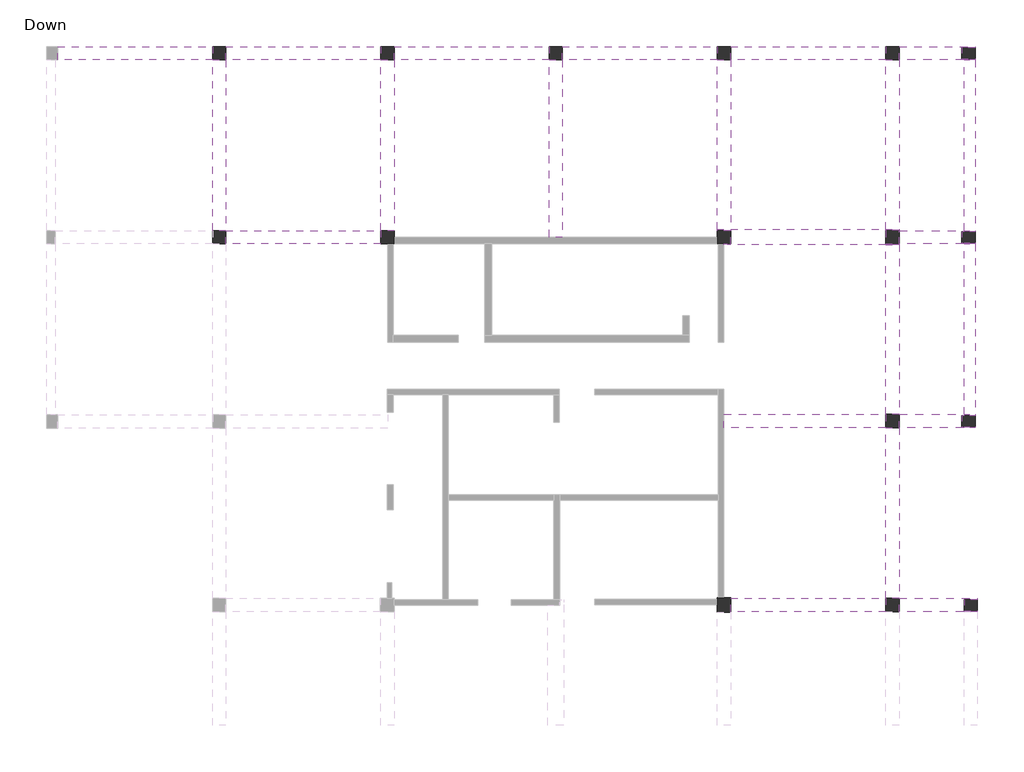
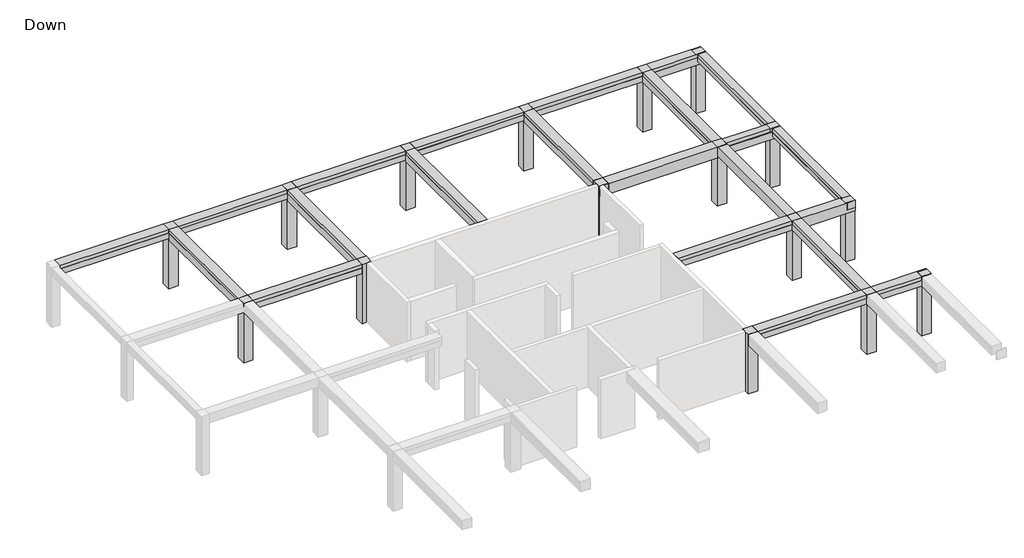
# One storey, part 2 of 2: 22 beams, 16 columns.
"""IFC4 building model written with IfcOpenShell, lengths in millimetres."""

from ifc_helpers import new_model, si_unit, frame, origin, origin_with_axes, place, context, project, spatial, polyline, outline, extrude, faceted_brep, element, save

model = new_model("IFC4")

# Units and contexts
model_context = context("Model", 3, world=origin())
ifc_project = project(units=[si_unit("LENGTHUNIT", "METRE", prefix="MILLI")], contexts=[model_context])

# Site, building, storey
site = spatial("IfcSite", under=ifc_project)
building = spatial("IfcBuilding", under=site)
storey = spatial("IfcBuildingStorey", under=building, Name="Down", Elevation=0.0)

# Beams
placement = place(None, origin())
element("IfcBeam", 1, ObjectType="Concrete Rectengular Beam : 50/50", at=placement, inside=storey, context=model_context, shape_type="Brep", body=[
    faceted_brep([(20278.3855721, 17336.6191558, 4000.0), (20278.3855721, 17386.6191558, 4000.0), (19788.3855721, 17386.6191558, 4000.0), (19788.3855721, 17336.6191558, 4000.0), (19778.3855721, 17386.6191558, 3500.0), (19778.3855721, 17336.6191558, 3500.0), (19778.3855721, 17336.6191558, 3770.0), (19778.3855721, 17386.6191558, 3770.0), (20278.3855721, 17336.6191558, 3500.0), (20278.3855721, 17386.6191558, 3500.0), (19788.3855721, 17336.6191558, 3770.0), (19788.3855721, 17386.6191558, 3770.0)], [[[0, 1, 2, 3]], [[4, 5, 6, 7]], [[8, 5, 4, 9]], [[0, 8, 9, 1]], [[5, 8, 0, 3, 10, 6]], [[9, 4, 7, 11, 2, 1]], [[10, 11, 7, 6]], [[11, 10, 3, 2]]]),
    faceted_brep([(20278.3855721, 25592.9632364, 3500.0), (19778.3855721, 25592.9632364, 3500.0), (19778.3855721, 25592.9632364, 3770.0), (19788.3855721, 25592.9632364, 3770.0), (19788.3855721, 25592.9632364, 4000.0), (20278.3855721, 25592.9632364, 4000.0), (19778.3855721, 17936.6191558, 3770.0), (19778.3855721, 17886.6191558, 3770.0), (19788.3855721, 17886.6191558, 3770.0), (19788.3855721, 17886.6191558, 4000.0), (20278.3855721, 17886.6191558, 4000.0), (19778.3855721, 17886.6191558, 3500.0), (20278.3855721, 17886.6191558, 3500.0), (19778.3855721, 17936.6191558, 3500.0), (20278.3855721, 17936.6191558, 3500.0)], [[[0, 1, 2, 3, 4, 5]], [[3, 2, 6, 7, 8]], [[4, 3, 8, 9]], [[10, 9, 8, 7, 11, 12]], [[10, 5, 4, 9]], [[1, 13, 11, 7, 6, 2]], [[1, 0, 14, 12, 11, 13]], [[0, 5, 10, 12, 14]]]),
])
element("IfcBeam", 2, ObjectType="Concrete Rectengular Beam : 50/50", at=placement, inside=storey, context=model_context, shape_type="Brep", body=[
    faceted_brep([(19778.3855721, 9081.6131842, 4000.0), (20278.3855721, 9081.6131842, 4000.0), (20278.3855721, 9131.6131842, 4000.0), (19778.3855721, 9131.6131842, 4000.0), (19778.3855721, 9081.6131842, 3500.0), (19778.3855721, 9131.6131842, 3500.0), (20278.3855721, 9081.6131842, 3500.0), (20278.3855721, 9131.6131842, 3500.0)], [[[0, 1, 2, 3]], [[4, 0, 3, 5]], [[6, 4, 5, 7]], [[1, 6, 7, 2]], [[1, 0, 4, 6]], [[3, 2, 7, 5]]]),
    faceted_brep([(20278.3855721, 9631.6131842, 4000.0), (19778.3855721, 9631.6131842, 4000.0), (19778.3855721, 9631.6131842, 3500.0), (20278.3855721, 9631.6131842, 3500.0), (20278.3855721, 17336.6191558, 4000.0), (19788.3855721, 17336.6191558, 4000.0), (19788.3855721, 9676.6131842, 4000.0), (19778.3855721, 9676.6131842, 4000.0), (19778.3855721, 9676.6131842, 3770.0), (19778.3855721, 9681.6131842, 3770.0), (19778.3855721, 17336.6191558, 3770.0), (19778.3855721, 17336.6191558, 3500.0), (19778.3855721, 9681.6131842, 3500.0), (20278.3855721, 17336.6191558, 3500.0), (20278.3855721, 9681.6131842, 3500.0), (19788.3855721, 17336.6191558, 3770.0), (19788.3855721, 9676.6131842, 3770.0)], [[[0, 1, 2, 3]], [[1, 0, 4, 5, 6, 7]], [[2, 1, 7, 8, 9, 10, 11, 12]], [[3, 2, 12, 11, 13, 14]], [[0, 3, 14, 13, 4]], [[13, 11, 10, 15, 5, 4]], [[8, 16, 15, 10, 9]], [[16, 6, 5, 15]], [[6, 16, 8, 7]]]),
])
element("IfcBeam", 3, ObjectType="Concrete Rectengular Beam : 60/60", at=placement, inside=storey, context=model_context, shape_type="SweptSolid", body=[
    extrude(outline(polyline([(26192.9632364, 3400.0), (25592.9632364, 3400.0), (25592.9632364, 3770.0), (25597.9632364, 3770.0), (25597.9632364, 4000.0), (26192.9632364, 4000.0), (26192.9632364, 3400.0)])), frame((-20894.7160223, 0.0, 0.0), z_axis=(1.0, 0.0, 0.0), x_axis=(0.0, 1.0, 0.0)), (0.0, 0.0, 1.0), 6950.9015474),
])
element("IfcBeam", 4, ObjectType="Concrete Rectengular Beam : 60/60", at=placement, inside=storey, context=model_context, shape_type="SweptSolid", body=[
    extrude(outline(polyline([(26192.9632364, 3400.0), (25592.9632364, 3400.0), (25592.9632364, 3770.0), (25597.9632364, 3770.0), (25597.9632364, 4000.0), (26192.9632364, 4000.0), (26192.9632364, 3400.0)])), frame((-13343.8144749, 0.0, 0.0), z_axis=(1.0, 0.0, 0.0), x_axis=(0.0, 1.0, 0.0)), (0.0, 0.0, 1.0), 6953.6558928),
])
element("IfcBeam", 5, ObjectType="Concrete Rectengular Beam : 60/60", at=placement, inside=storey, context=model_context, shape_type="SweptSolid", body=[
    extrude(outline(polyline([(26192.9632364, 3400.0), (25592.9632364, 3400.0), (25592.9632364, 3770.0), (25597.9632364, 3770.0), (25597.9632364, 4000.0), (26192.9632364, 4000.0), (26192.9632364, 3400.0)])), frame((-5790.1585821, 0.0, 0.0), z_axis=(1.0, 0.0, 0.0), x_axis=(0.0, 1.0, 0.0)), (0.0, 0.0, 1.0), 6947.2395979),
])
element("IfcBeam", 6, ObjectType="Concrete Rectengular Beam : 60/60", at=placement, inside=storey, context=model_context, shape_type="SweptSolid", body=[
    extrude(outline(polyline([(26192.9632364, 3400.0), (25592.9632364, 3400.0), (25592.9632364, 3770.0), (25597.9632364, 3770.0), (25597.9632364, 4000.0), (26192.9632364, 4000.0), (26192.9632364, 3400.0)])), frame((1757.0810158, 0.0, 0.0), z_axis=(1.0, 0.0, 0.0), x_axis=(0.0, 1.0, 0.0)), (0.0, 0.0, 1.0), 6946.2785308),
])
element("IfcBeam", 7, ObjectType="Concrete Rectengular Beam : 60/60", at=placement, inside=storey, context=model_context, shape_type="SweptSolid", body=[
    extrude(outline(polyline([(26192.9632364, 3400.0), (25592.9632364, 3400.0), (25592.9632364, 3770.0), (25597.9632364, 3770.0), (25597.9632364, 4000.0), (26192.9632364, 4000.0), (26192.9632364, 3400.0)])), frame((9303.3595467, 0.0, 0.0), z_axis=(1.0, 0.0, 0.0), x_axis=(0.0, 1.0, 0.0)), (0.0, 0.0, 1.0), 6958.5206647),
])
element("IfcBeam", 8, ObjectType="Concrete Rectengular Beam : 60/60", at=placement, inside=storey, context=model_context, shape_type="SweptSolid", body=[
    extrude(outline(polyline([(3400.0, 16261.8802114), (3400.0, 16861.8802114), (4000.0, 16861.8802114), (4000.0, 16266.8802114), (3770.0, 16266.8802114), (3770.0, 16261.8802114), (3400.0, 16261.8802114)])), frame((0.0, 1432.5009852, 0.0), z_axis=(0.0, 1.0, 0.0), x_axis=(0.0, 0.0, 1.0)), (0.0, 0.0, 1.0), 7649.112199),
])
element("IfcBeam", 9, ObjectType="Concrete Rectengular Beam : 60/60", at=placement, inside=storey, context=model_context, shape_type="SweptSolid", body=[
    extrude(outline(polyline([(1432.5009852, 3400.0), (832.5009852, 3400.0), (832.5009852, 3770.0), (837.5009852, 3770.0), (837.5009852, 4000.0), (1427.5009852, 4000.0), (1427.5009852, 3770.0), (1432.5009852, 3770.0), (1432.5009852, 3400.0)])), frame((9303.3595467, 0.0, 0.0), z_axis=(1.0, 0.0, 0.0), x_axis=(0.0, 1.0, 0.0)), (0.0, 0.0, 1.0), 6958.5206647),
])
element("IfcBeam", 10, ObjectType="Concrete Rectengular Beam : 60/60", at=placement, inside=storey, context=model_context, shape_type="SweptSolid", body=[
    extrude(outline(polyline([(17936.6191558, 3400.0), (17336.6191558, 3400.0), (17336.6191558, 3770.0), (17341.6191558, 3770.0), (17341.6191558, 4000.0), (17931.6191558, 4000.0), (17931.6191558, 3770.0), (17936.6191558, 3770.0), (17936.6191558, 3400.0)])), frame((-13343.8144749, 0.0, 0.0), z_axis=(1.0, 0.0, 0.0), x_axis=(0.0, 1.0, 0.0)), (0.0, 0.0, 1.0), 6953.6558928),
])
element("IfcBeam", 11, ObjectType="Concrete Rectengular Beam : 60/60", at=placement, inside=storey, context=model_context, shape_type="Brep", body=[
    faceted_brep([(16261.8802114, 9086.6131842, 4000.0), (16261.8802114, 9681.6131842, 4000.0), (9006.9599651, 9681.6131842, 4000.0), (9006.9599651, 9086.6131842, 4000.0), (16261.8802114, 9681.6131842, 3770.0), (16261.8802114, 9681.6131842, 3400.0), (9006.9599651, 9681.6131842, 3400.0), (9006.9599651, 9681.6131842, 3770.0), (16261.8802114, 9081.6131842, 3400.0), (9006.9599651, 9081.6131842, 3400.0), (16261.8802114, 9081.6131842, 3770.0), (9006.9599651, 9081.6131842, 3770.0), (16261.8802114, 9086.6131842, 3770.0), (9006.9599651, 9086.6131842, 3770.0)], [[[0, 1, 2, 3]], [[1, 4, 5, 6, 7, 2]], [[5, 8, 9, 6]], [[8, 10, 11, 9]], [[5, 4, 1, 0, 12, 10, 8]], [[10, 12, 13, 11]], [[12, 0, 3, 13]], [[3, 2, 7, 6, 9, 11, 13]]]),
])
element("IfcBeam", 12, ObjectType="Concrete Rectengular Beam : 60/60", at=placement, inside=storey, context=model_context, shape_type="Brep", body=[
    faceted_brep([(16261.8802114, 17293.0356779, 4000.0), (16261.8802114, 9681.6131842, 4000.0), (16856.8802114, 9681.6131842, 4000.0), (16856.8802114, 17293.0356779, 4000.0), (16861.8802114, 9681.6131842, 3400.0), (16861.8802114, 17293.0356779, 3400.0), (16861.8802114, 17293.0356779, 3770.0), (16861.8802114, 9681.6131842, 3770.0), (16261.8802114, 17293.0356779, 3400.0), (16261.8802114, 9681.6131842, 3400.0), (16261.8802114, 9681.6131842, 3770.0), (16261.8802114, 17293.0356779, 3770.0), (16856.8802114, 9681.6131842, 3770.0), (16856.8802114, 17293.0356779, 3770.0)], [[[0, 1, 2, 3]], [[4, 5, 6, 7]], [[8, 5, 4, 9]], [[9, 10, 1, 0, 11, 8]], [[1, 10, 9, 4, 7, 12, 2]], [[5, 8, 11, 0, 3, 13, 6]], [[13, 12, 7, 6]], [[12, 13, 3, 2]]]),
])
element("IfcBeam", 13, ObjectType="Concrete Rectengular Beam : 60/60", at=placement, inside=storey, context=model_context, shape_type="Brep", body=[
    faceted_brep([(20381.7521333, 1432.5009852, 4000.0), (16861.8802114, 1432.5009852, 4000.0), (16861.8802114, 837.5009852, 4000.0), (19786.5095237, 837.5009852, 4000.0), (19786.5074854, 832.5009852, 4000.0), (20381.5075349, 832.5009852, 4000.0), (20381.5197648, 862.5009852, 4000.0), (19781.6298091, 862.5009852, 4000.0), (19781.6298091, 1362.5009852, 4000.0), (20381.7235968, 1362.5009852, 4000.0), (20381.5075349, 832.5009852, 3400.0), (19786.5074854, 832.5009852, 3770.0), (16861.8802114, 832.5009852, 3770.0), (16861.8802114, 832.5009852, 3400.0), (19781.507485, 832.5009852, 3400.0), (16861.8802114, 1432.5009852, 3400.0), (20381.7521333, 1432.5009852, 3400.0), (20381.7235968, 1362.5009852, 3400.0), (19781.6298091, 1362.5009852, 3400.0), (19781.6298091, 862.5009852, 3400.0), (20381.5197648, 862.5009852, 3400.0), (16861.8802114, 837.5009852, 3770.0), (19786.5095237, 837.5009852, 3770.0)], [[[0, 1, 2, 3, 4, 5, 6, 7, 8, 9]], [[10, 5, 4, 11, 12, 13, 14]], [[15, 16, 17, 18, 19, 20, 10, 14, 13]], [[15, 1, 0, 16]], [[1, 15, 13, 12, 21, 2]], [[22, 21, 12, 11]], [[3, 22, 11, 4]], [[22, 3, 2, 21]], [[16, 0, 9, 17]], [[19, 7, 6, 20]], [[7, 19, 18, 8]], [[8, 18, 17, 9]], [[5, 10, 20, 6]]]),
])
element("IfcBeam", 14, ObjectType="Concrete Rectengular Beam : 60/65", at=placement, inside=storey, context=model_context, shape_type="Brep", body=[
    faceted_brep([(9303.3595467, 17293.0356779, 4000.0), (9303.3595467, 17336.6191558, 4000.0), (9006.9599651, 17336.6191558, 4000.0), (9006.9599651, 17293.0356779, 4000.0), (9303.3595467, 17293.0356779, 3350.0), (9303.3595467, 17336.6191558, 3350.0), (9006.9599651, 17293.0356779, 3770.0), (9006.9599651, 17293.0356779, 3350.0), (9006.9599651, 17336.6191558, 3350.0)], [[[0, 1, 2, 3]], [[0, 4, 5, 1]], [[4, 0, 3, 6, 7]], [[3, 2, 8, 7, 6]], [[5, 4, 7, 8]], [[1, 5, 8, 2]]]),
    faceted_brep([(8703.3595467, 17336.6191558, 3350.0), (8703.3595467, 17293.0356779, 3350.0), (8703.3595467, 17293.0356779, 3770.0), (8703.3595467, 17336.6191558, 3770.0), (8756.9599651, 17336.6191558, 3350.0), (8756.9599651, 17293.0356779, 3350.0), (8756.9599651, 17336.6191558, 3770.0), (8756.9599651, 17293.0356779, 3770.0)], [[[0, 1, 2, 3]], [[1, 0, 4, 5]], [[0, 3, 6, 4]], [[3, 2, 7, 6]], [[5, 4, 6, 7]], [[2, 1, 5, 7]]]),
    faceted_brep([(9303.3595467, 25592.9632364, 3350.0), (8703.3595467, 25592.9632364, 3350.0), (8703.3595467, 25592.9632364, 3770.0), (8708.3595467, 25592.9632364, 3770.0), (8708.3595467, 25592.9632364, 4000.0), (9298.3595467, 25592.9632364, 4000.0), (9298.3595467, 25592.9632364, 3770.0), (9303.3595467, 25592.9632364, 3770.0), (8703.3595467, 17936.6191558, 3350.0), (9303.3595467, 17936.6191558, 3350.0), (9303.3595467, 17936.6191558, 4000.0), (8708.3595467, 17936.6191558, 4000.0), (8708.3595467, 17936.6191558, 3770.0), (8703.3595467, 17936.6191558, 3770.0), (9303.3595467, 17938.0356779, 4000.0), (9298.3595467, 17938.0356779, 4000.0), (8703.3595467, 17993.0356779, 3350.0), (9303.3595467, 17993.0356779, 3350.0), (9303.3595467, 17993.0356779, 3770.0), (9303.3595467, 17938.0356779, 3770.0), (9298.3595467, 17938.0356779, 3770.0)], [[[0, 1, 2, 3, 4, 5, 6, 7]], [[8, 9, 10, 11, 12, 13]], [[11, 10, 14, 15, 5, 4]], [[1, 16, 8, 13, 2]], [[1, 0, 17, 9, 8, 16]], [[10, 9, 17, 0, 7, 18, 19, 14]], [[6, 20, 19, 18, 7]], [[20, 15, 14, 19]], [[15, 20, 6, 5]], [[12, 3, 2, 13]], [[3, 12, 11, 4]]]),
])
element("IfcBeam", 15, ObjectType="Concrete Rectengular Beam : 60/65", at=placement, inside=storey, context=model_context, shape_type="Brep", body=[
    faceted_brep([(16261.8802114, 17343.0356779, 4000.0), (16261.8802114, 17293.0356779, 4000.0), (16856.8802114, 17293.0356779, 4000.0), (16856.8802114, 17343.0356779, 4000.0), (16261.8802114, 17293.0356779, 3350.0), (16261.8802114, 17293.0356779, 3400.0), (16261.8802114, 17343.0356779, 3350.0), (16861.8802114, 17293.0356779, 3350.0), (16861.8802114, 17343.0356779, 3350.0), (16861.8802114, 17343.0356779, 3770.0), (16861.8802114, 17336.6191558, 3770.0), (16861.8802114, 17293.0356779, 3770.0), (16861.8802114, 17293.0356779, 3400.0), (16856.8802114, 17293.0356779, 3770.0), (16856.8802114, 17343.0356779, 3770.0)], [[[0, 1, 2, 3]], [[4, 5, 1, 0, 6]], [[7, 4, 6, 8]], [[7, 8, 9, 10, 11, 12]], [[1, 5, 4, 7, 12, 11, 13, 2]], [[6, 0, 3, 14, 9, 8]], [[14, 13, 11, 10, 9]], [[13, 14, 3, 2]]]),
    faceted_brep([(16861.8802114, 25592.9632364, 3350.0), (16261.8802114, 25592.9632364, 3350.0), (16261.8802114, 25592.9632364, 3770.0), (16266.8802114, 25592.9632364, 3770.0), (16266.8802114, 25592.9632364, 4000.0), (16856.8802114, 25592.9632364, 4000.0), (16856.8802114, 25592.9632364, 3770.0), (16861.8802114, 25592.9632364, 3770.0), (16261.8802114, 17943.0356779, 3350.0), (16861.8802114, 17943.0356779, 3350.0), (16861.8802114, 17943.0356779, 3770.0), (16856.8802114, 17943.0356779, 3770.0), (16856.8802114, 17943.0356779, 4000.0), (16266.8802114, 17943.0356779, 4000.0), (16266.8802114, 17943.0356779, 3770.0), (16261.8802114, 17943.0356779, 3770.0), (16261.8802114, 17993.0356779, 3350.0), (16261.8802114, 17993.0356779, 3770.0), (16861.8802114, 17993.0356779, 3350.0)], [[[0, 1, 2, 3, 4, 5, 6, 7]], [[8, 9, 10, 11, 12, 13, 14, 15]], [[4, 13, 12, 5]], [[1, 16, 8, 15, 17, 2]], [[1, 0, 18, 9, 8, 16]], [[9, 18, 0, 7, 10]], [[14, 3, 2, 17, 15]], [[3, 14, 13, 4]], [[6, 11, 10, 7]], [[11, 6, 5, 12]]]),
])
element("IfcBeam", 16, ObjectType="Concrete Rectengular Beam : 60/70", at=placement, inside=storey, context=model_context, shape_type="SweptSolid", body=[
    extrude(outline(polyline([(3300.0, -6390.1585821), (3300.0, -5790.1585821), (3770.0, -5790.1585821), (3770.0, -5795.1585821), (4000.0, -5795.1585821), (4000.0, -6385.1585821), (3770.0, -6385.1585821), (3770.0, -6390.1585821), (3300.0, -6390.1585821)])), frame((0.0, 17936.6191558, 0.0), z_axis=(0.0, 1.0, 0.0), x_axis=(0.0, 0.0, 1.0)), (0.0, 0.0, 1.0), 7656.3440805),
])
element("IfcBeam", 17, ObjectType="Concrete Rectengular Beam : 60/70", at=placement, inside=storey, context=model_context, shape_type="SweptSolid", body=[
    extrude(outline(polyline([(3300.0, -13943.8144749), (3300.0, -13343.8144749), (3770.0, -13343.8144749), (3770.0, -13348.8144749), (4000.0, -13348.8144749), (4000.0, -13938.8144749), (3770.0, -13938.8144749), (3770.0, -13943.8144749), (3300.0, -13943.8144749)])), frame((0.0, 17936.6191558, 0.0), z_axis=(0.0, 1.0, 0.0), x_axis=(0.0, 0.0, 1.0)), (0.0, 0.0, 1.0), 7656.3440805),
])
element("IfcBeam", 18, ObjectType="Concrete Rectengular Beam : 60/70", at=placement, inside=storey, context=model_context, shape_type="SweptSolid", body=[
    extrude(outline(polyline([(4000.0, 1752.0810158), (4000.0, 1162.0810158), (3770.0, 1162.0810158), (3770.0, 1157.0810158), (3300.0, 1157.0810158), (3300.0, 1757.0810158), (3770.0, 1757.0810158), (3770.0, 1752.0810158), (4000.0, 1752.0810158)])), frame((0.0, 17636.6191558, 0.0), z_axis=(0.0, 1.0, 0.0), x_axis=(0.0, 0.0, 1.0)), (0.0, 0.0, 1.0), 7956.3440805),
])
element("IfcBeam", 19, ObjectType="Concrete Rectengular Beam : 60/70", at=placement, inside=storey, context=model_context, shape_type="Brep", body=[
    faceted_brep([(20278.3855721, 26192.9632364, 4000.0), (16861.8802114, 26192.9632364, 4000.0), (16861.8802114, 25597.9632364, 4000.0), (19788.3855721, 25597.9632364, 4000.0), (19788.3855721, 25592.9632364, 4000.0), (20278.3855721, 25592.9632364, 4000.0), (20278.3855721, 25642.9632364, 4000.0), (19678.3855721, 25642.9632364, 4000.0), (19678.3855721, 26142.9632364, 4000.0), (20278.3855721, 26142.9632364, 4000.0), (20278.3855721, 25592.9632364, 3300.0), (20278.3855721, 25592.9632364, 3500.0), (19788.3855721, 25592.9632364, 3770.0), (19778.3855721, 25592.9632364, 3770.0), (16861.8802114, 25592.9632364, 3770.0), (16861.8802114, 25592.9632364, 3300.0), (16861.8802114, 26192.9632364, 3300.0), (20278.3855721, 26192.9632364, 3300.0), (20278.3855721, 26142.9632364, 3300.0), (19678.3855721, 26142.9632364, 3300.0), (19678.3855721, 25642.9632364, 3300.0), (20278.3855721, 25642.9632364, 3300.0), (16861.8802114, 25597.9632364, 3770.0), (19788.3855721, 25597.9632364, 3770.0)], [[[0, 1, 2, 3, 4, 5, 6, 7, 8, 9]], [[10, 11, 5, 4, 12, 13, 14, 15]], [[15, 16, 17, 18, 19, 20, 21, 10]], [[16, 1, 0, 17]], [[16, 15, 14, 22, 2, 1]], [[23, 22, 14, 13, 12]], [[3, 23, 12, 4]], [[23, 3, 2, 22]], [[17, 0, 9, 18]], [[20, 7, 6, 21]], [[7, 20, 19, 8]], [[8, 19, 18, 9]], [[5, 11, 10, 21, 6]]]),
])
element("IfcBeam", 20, ObjectType="Concrete Rectengular Beam : 60/70", at=placement, inside=storey, context=model_context, shape_type="Brep", body=[
    faceted_brep([(19678.3855721, 17863.0356779, 4000.0), (16861.8802114, 17863.0356779, 4000.0), (16861.8802114, 17396.6191558, 4000.0), (19678.3855721, 17396.6191558, 4000.0), (20278.3855721, 17936.6191558, 3300.0), (16861.8802114, 17936.6191558, 3300.0), (16861.8802114, 17936.6191558, 3770.0), (19778.3855721, 17936.6191558, 3770.0), (19778.3855721, 17936.6191558, 3500.0), (20278.3855721, 17936.6191558, 3500.0), (16861.8802114, 17336.6191558, 3300.0), (16861.8802114, 17343.0356779, 3300.0), (20278.3855721, 17886.6191558, 3300.0), (19678.3855721, 17886.6191558, 3300.0), (19678.3855721, 17386.6191558, 3300.0), (20278.3855721, 17386.6191558, 3300.0), (20278.3855721, 17336.6191558, 3300.0), (20278.3855721, 17336.6191558, 3500.0), (19778.3855721, 17336.6191558, 3500.0), (19778.3855721, 17336.6191558, 3770.0), (16861.8802114, 17336.6191558, 3770.0), (16861.8802114, 17343.0356779, 3770.0), (16861.8802114, 17396.6191558, 3770.0), (16861.8802114, 17863.0356779, 3770.0), (19678.3855721, 17863.0356779, 3770.0), (19678.3855721, 17886.6191558, 3770.0), (19778.3855721, 17886.6191558, 3770.0), (20278.3855721, 17886.6191558, 3500.0), (19678.3855721, 17386.6191558, 3770.0), (19778.3855721, 17386.6191558, 3770.0), (19778.3855721, 17386.6191558, 3500.0), (20278.3855721, 17386.6191558, 3500.0), (19678.3855721, 17396.6191558, 3770.0), (19778.3855721, 17886.6191558, 3500.0)], [[[0, 1, 2, 3]], [[4, 5, 6, 7, 8, 9]], [[10, 11, 5, 4, 12, 13, 14, 15, 16]], [[10, 16, 17, 18, 19, 20]], [[5, 11, 10, 20, 21, 22, 2, 1, 23, 6]], [[6, 23, 24, 25, 26, 7]], [[23, 1, 0, 24]], [[12, 4, 9, 27]], [[15, 14, 28, 29, 30, 31]], [[14, 13, 25, 24, 0, 3, 32, 28]], [[13, 12, 27, 33, 26, 25]], [[16, 15, 31, 17]], [[32, 22, 21, 20, 19, 29, 28]], [[22, 32, 3, 2]], [[18, 30, 29, 19]], [[30, 18, 17, 31]], [[33, 8, 7, 26]], [[8, 33, 27, 9]]]),
])
element("IfcBeam", 21, ObjectType="Concrete Rectengular Beam : 60/70", at=placement, inside=storey, context=model_context, shape_type="Brep", body=[
    faceted_brep([(19678.3855721, 9131.6131842, 4000.0), (19678.3855721, 9631.6131842, 4000.0), (19778.3855721, 9631.6131842, 4000.0), (19778.3855721, 9676.6131842, 4000.0), (16861.8802114, 9676.6131842, 4000.0), (16861.8802114, 9081.6131842, 4000.0), (19778.3855721, 9081.6131842, 4000.0), (19778.3855721, 9131.6131842, 4000.0), (20278.3855721, 9681.6131842, 3300.0), (16861.8802114, 9681.6131842, 3300.0), (16861.8802114, 9681.6131842, 3770.0), (19778.3855721, 9681.6131842, 3770.0), (19778.3855721, 9681.6131842, 3500.0), (20278.3855721, 9681.6131842, 3500.0), (16861.8802114, 9081.6131842, 3300.0), (20278.3855721, 9631.6131842, 3300.0), (19678.3855721, 9631.6131842, 3300.0), (19678.3855721, 9131.6131842, 3300.0), (20278.3855721, 9131.6131842, 3300.0), (20278.3855721, 9081.6131842, 3300.0), (20278.3855721, 9081.6131842, 3500.0), (19778.3855721, 9081.6131842, 3500.0), (16861.8802114, 9676.6131842, 3770.0), (20278.3855721, 9631.6131842, 3500.0), (19778.3855721, 9131.6131842, 3500.0), (20278.3855721, 9131.6131842, 3500.0), (19778.3855721, 9631.6131842, 3500.0), (19778.3855721, 9676.6131842, 3770.0)], [[[0, 1, 2, 3, 4, 5, 6, 7]], [[8, 9, 10, 11, 12, 13]], [[14, 9, 8, 15, 16, 17, 18, 19]], [[14, 19, 20, 21, 6, 5]], [[9, 14, 5, 4, 22, 10]], [[15, 8, 13, 23]], [[17, 0, 7, 24, 25, 18]], [[0, 17, 16, 1]], [[1, 16, 15, 23, 26, 2]], [[19, 18, 25, 20]], [[10, 22, 27, 11]], [[22, 4, 3, 27]], [[21, 24, 7, 6]], [[24, 21, 20, 25]], [[26, 12, 11, 27, 3, 2]], [[12, 26, 23, 13]]]),
])
element("IfcBeam", 22, ObjectType="Concrete Rectengular Beam : 70/70", at=placement, inside=storey, context=model_context, shape_type="Brep", body=[
    faceted_brep([(9303.3595467, 17938.0356779, 4000.0), (9303.3595467, 17936.6191558, 4000.0), (9303.3595467, 17336.6191558, 4000.0), (9303.3595467, 17293.0356779, 4000.0), (16261.8802114, 17293.0356779, 4000.0), (16261.8802114, 17343.0356779, 4000.0), (16261.8802114, 17938.0356779, 4000.0), (16861.8802114, 17993.0356779, 3300.0), (8703.3595467, 17993.0356779, 3300.0), (8703.3595467, 17993.0356779, 3350.0), (9303.3595467, 17993.0356779, 3350.0), (9303.3595467, 17993.0356779, 3770.0), (16261.8802114, 17993.0356779, 3770.0), (16261.8802114, 17993.0356779, 3350.0), (16861.8802114, 17993.0356779, 3350.0), (16861.8802114, 17943.0356779, 3300.0), (16861.8802114, 17943.0356779, 3350.0), (8703.3595467, 17936.6191558, 3300.0), (8703.3595467, 17936.6191558, 3350.0), (16861.8802114, 17343.0356779, 3300.0), (16261.8802114, 17343.0356779, 3300.0), (16261.8802114, 17343.0356779, 3350.0), (16861.8802114, 17343.0356779, 3350.0), (16261.8802114, 17943.0356779, 3300.0), (16261.8802114, 17943.0356779, 3350.0), (16261.8802114, 17943.0356779, 3770.0), (16261.8802114, 17939.0120642, 3770.0), (16261.8802114, 17938.0356779, 3770.0), (16261.8802114, 17293.0356779, 3770.0), (16261.8802114, 17293.0356779, 3400.0), (16261.8802114, 17293.0356779, 3350.0), (16861.8802114, 17293.0356779, 3300.0), (16861.8802114, 17336.6191558, 3300.0), (16861.8802114, 17293.0356779, 3350.0), (9303.3595467, 17936.6191558, 3300.0), (9303.3595467, 17336.6191558, 3300.0), (9303.3595467, 17336.6191558, 3350.0), (9303.3595467, 17293.0356779, 3350.0), (9303.3595467, 17938.0356779, 3770.0), (9303.3595467, 17936.6191558, 3350.0), (9006.9599651, 17336.6191558, 3300.0), (9006.9599651, 17293.0356779, 3300.0), (9006.9599651, 17293.0356779, 3350.0), (9006.9599651, 17336.6191558, 3350.0)], [[[0, 1, 2, 3, 4, 5, 6]], [[7, 8, 9, 10, 11, 12, 13, 14]], [[15, 7, 14, 16]], [[8, 17, 18, 9]], [[19, 20, 21, 22]], [[20, 23, 24, 13, 12, 25, 26, 27, 6, 5, 4, 28, 29, 30, 21]], [[23, 15, 16, 24]], [[31, 32, 19, 22, 33]], [[34, 35, 36, 37, 3, 2, 1, 0, 38, 11, 10, 39]], [[17, 34, 39, 18]], [[38, 27, 26, 25, 12, 11]], [[6, 27, 38, 0]], [[39, 10, 9, 18]], [[21, 30, 33, 22]], [[13, 24, 16, 14]], [[40, 41, 42, 43]], [[8, 7, 15, 23, 20, 19, 32, 31, 41, 40, 35, 34, 17]], [[3, 37, 42, 41, 31, 33, 30, 29, 28, 4]], [[36, 35, 40, 43]], [[37, 36, 43, 42]]]),
    faceted_brep([(8703.3595467, 17293.0356779, 3300.0), (8703.3595467, 17336.6191558, 3300.0), (8756.9599651, 17336.6191558, 3300.0), (8756.9599651, 17293.0356779, 3300.0), (8703.3595467, 17293.0356779, 3350.0), (8756.9599651, 17293.0356779, 3350.0), (8703.3595467, 17336.6191558, 3350.0), (8756.9599651, 17336.6191558, 3350.0)], [[[0, 1, 2, 3]], [[4, 0, 3, 5]], [[1, 6, 7, 2]], [[1, 0, 4, 6]], [[6, 4, 5, 7]], [[3, 2, 7, 5]]]),
])

# Columns
element("IfcColumn", 23, ObjectType="Concrete Rectengular Column : 60/50", at=placement, inside=storey, context=model_context, shape_type="Brep", body=[
    faceted_brep([(20381.6298091, 1362.5009852, 0.0), (20381.6298091, 862.5009852, 0.0), (19781.6298091, 862.5009852, 0.0), (19781.6298091, 1362.5009852, 0.0), (20381.6298091, 1362.5009852, 4000.0), (20381.6298091, 862.5009852, 4000.0), (19781.6298091, 862.5009852, 4000.0), (19781.6298091, 862.5009852, 3400.0), (19781.6298091, 1362.5009852, 4000.0), (19781.6298091, 1362.5009852, 3400.0)], [[[0, 1, 2, 3]], [[4, 5, 1, 0]], [[5, 6, 7, 2, 1]], [[6, 8, 9, 3, 2, 7]], [[8, 4, 0, 3, 9]], [[4, 8, 6, 5]]]),
])
element("IfcColumn", 24, ObjectType="Concrete Rectengular Column : 60/50", at=placement, inside=storey, context=model_context, shape_type="SweptSolid", body=[
    extrude(outline(polyline([(20278.3855721, 9631.6131842), (20278.3855721, 9131.6131842), (19678.3855721, 9131.6131842), (19678.3855721, 9631.6131842), (20278.3855721, 9631.6131842)])), origin_with_axes(), (0.0, 0.0, 1.0), 4000.0),
])
element("IfcColumn", 25, ObjectType="Concrete Rectengular Column : 60/50", at=placement, inside=storey, context=model_context, shape_type="Brep", body=[
    faceted_brep([(20278.3855721, 17886.6191558, 0.0), (20278.3855721, 17386.6191558, 0.0), (19678.3855721, 17386.6191558, 0.0), (19678.3855721, 17886.6191558, 0.0), (20278.3855721, 17886.6191558, 4000.0), (20278.3855721, 17386.6191558, 4000.0), (20278.3855721, 17386.6191558, 3500.0), (20278.3855721, 17386.6191558, 3300.0), (20278.3855721, 17886.6191558, 3300.0), (20278.3855721, 17886.6191558, 3500.0), (19788.3855721, 17386.6191558, 4000.0), (19678.3855721, 17386.6191558, 4000.0), (19678.3855721, 17386.6191558, 3770.0), (19678.3855721, 17386.6191558, 3300.0), (19678.3855721, 17396.6191558, 4000.0), (19678.3855721, 17863.0356779, 4000.0), (19678.3855721, 17886.6191558, 4000.0), (19678.3855721, 17886.6191558, 3770.0), (19678.3855721, 17886.6191558, 3300.0), (19788.3855721, 17886.6191558, 4000.0)], [[[0, 1, 2, 3]], [[4, 5, 6, 7, 1, 0, 8, 9]], [[5, 10, 11, 12, 13, 2, 1, 7, 6]], [[11, 14, 15, 16, 17, 18, 3, 2, 13, 12]], [[16, 19, 4, 9, 8, 0, 3, 18, 17]], [[4, 19, 16, 15, 14, 11, 10, 5]]]),
])
element("IfcColumn", 26, ObjectType="Concrete Rectengular Column : 60/50", at=placement, inside=storey, context=model_context, shape_type="Brep", body=[
    faceted_brep([(20278.3855721, 26142.9632364, 0.0), (20278.3855721, 25642.9632364, 0.0), (19678.3855721, 25642.9632364, 0.0), (19678.3855721, 26142.9632364, 0.0), (20278.3855721, 26142.9632364, 4000.0), (20278.3855721, 25642.9632364, 4000.0), (20278.3855721, 25642.9632364, 3300.0), (20278.3855721, 26142.9632364, 3300.0), (19678.3855721, 25642.9632364, 4000.0), (19678.3855721, 25642.9632364, 3300.0), (19678.3855721, 26142.9632364, 4000.0), (19678.3855721, 26142.9632364, 3300.0)], [[[0, 1, 2, 3]], [[4, 5, 6, 1, 0, 7]], [[5, 8, 9, 2, 1, 6]], [[8, 10, 11, 3, 2, 9]], [[10, 4, 7, 0, 3, 11]], [[4, 10, 8, 5]]]),
])
element("IfcColumn", 27, ObjectType="Concrete Rectengular Column : 60/60", at=placement, inside=storey, context=model_context, shape_type="Brep", body=[
    faceted_brep([(-13343.8144749, 26192.9632364, 0.0), (-13343.8144749, 25592.9632364, 0.0), (-13943.8144749, 25592.9632364, 0.0), (-13943.8144749, 26192.9632364, 0.0), (-13343.8144749, 26192.9632364, 4000.0), (-13343.8144749, 25597.9632364, 4000.0), (-13343.8144749, 25592.9632364, 4000.0), (-13343.8144749, 25592.9632364, 3770.0), (-13348.8144749, 25592.9632364, 4000.0), (-13938.8144749, 25592.9632364, 4000.0), (-13943.8144749, 25592.9632364, 4000.0), (-13943.8144749, 25592.9632364, 3770.0), (-13943.8144749, 25597.9632364, 4000.0), (-13943.8144749, 26192.9632364, 4000.0)], [[[0, 1, 2, 3]], [[4, 5, 6, 7, 1, 0]], [[6, 8, 9, 10, 11, 2, 1, 7]], [[10, 12, 13, 3, 2, 11]], [[13, 4, 0, 3]], [[4, 13, 12, 10, 9, 8, 6, 5]]]),
])
element("IfcColumn", 28, ObjectType="Concrete Rectengular Column : 60/60", at=placement, inside=storey, context=model_context, shape_type="Brep", body=[
    faceted_brep([(-13343.8144749, 17936.6191558, 0.0), (-13343.8144749, 17336.6191558, 0.0), (-13943.8144749, 17336.6191558, 0.0), (-13943.8144749, 17936.6191558, 0.0), (-13343.8144749, 17936.6191558, 4000.0), (-13343.8144749, 17931.6191558, 4000.0), (-13343.8144749, 17341.6191558, 4000.0), (-13343.8144749, 17336.6191558, 4000.0), (-13343.8144749, 17336.6191558, 3770.0), (-13343.8144749, 17936.6191558, 3770.0), (-13348.8144749, 17336.6191558, 4000.0), (-13938.8144749, 17336.6191558, 4000.0), (-13943.8144749, 17336.6191558, 4000.0), (-13943.8144749, 17336.6191558, 3770.0), (-13943.8144749, 17341.6191558, 4000.0), (-13943.8144749, 17931.6191558, 4000.0), (-13943.8144749, 17936.6191558, 4000.0), (-13943.8144749, 17936.6191558, 3770.0), (-13938.8144749, 17936.6191558, 4000.0), (-13348.8144749, 17936.6191558, 4000.0)], [[[0, 1, 2, 3]], [[4, 5, 6, 7, 8, 1, 0, 9]], [[7, 10, 11, 12, 13, 2, 1, 8]], [[12, 14, 15, 16, 17, 3, 2, 13]], [[16, 18, 19, 4, 9, 0, 3, 17]], [[4, 19, 18, 16, 15, 14, 12, 11, 10, 7, 6, 5]]]),
])
element("IfcColumn", 29, ObjectType="Concrete Rectengular Column : 60/60", at=placement, inside=storey, context=model_context, shape_type="Brep", body=[
    faceted_brep([(-5790.1585821, 26192.9632364, 0.0), (-5790.1585821, 25592.9632364, 0.0), (-6390.1585821, 25592.9632364, 0.0), (-6390.1585821, 26192.9632364, 0.0), (-5790.1585821, 26192.9632364, 4000.0), (-5790.1585821, 25597.9632364, 4000.0), (-5790.1585821, 25592.9632364, 4000.0), (-5790.1585821, 25592.9632364, 3770.0), (-5795.1585821, 25592.9632364, 4000.0), (-6385.1585821, 25592.9632364, 4000.0), (-6390.1585821, 25592.9632364, 4000.0), (-6390.1585821, 25592.9632364, 3770.0), (-6390.1585821, 25597.9632364, 4000.0), (-6390.1585821, 26192.9632364, 4000.0)], [[[0, 1, 2, 3]], [[4, 5, 6, 7, 1, 0]], [[6, 8, 9, 10, 11, 2, 1, 7]], [[10, 12, 13, 3, 2, 11]], [[13, 4, 0, 3]], [[4, 13, 12, 10, 9, 8, 6, 5]]]),
])
element("IfcColumn", 30, ObjectType="Concrete Rectengular Column : 60/60", at=placement, inside=storey, context=model_context, shape_type="Brep", body=[
    faceted_brep([(-5790.1585821, 17336.6191558, 0.0), (-5840.1585821, 17336.6191558, 0.0), (-6090.1585821, 17336.6191558, 0.0), (-6390.1585821, 17336.6191558, 0.0), (-6390.1585821, 17936.6191558, 0.0), (-5790.1585821, 17936.6191558, 0.0), (-5790.1585821, 17636.6191558, 0.0), (-5790.1585821, 17336.6191558, 4000.0), (-5840.1585821, 17336.6191558, 4000.0), (-6090.1585821, 17336.6191558, 4000.0), (-6390.1585821, 17336.6191558, 4000.0), (-6390.1585821, 17336.6191558, 3770.0), (-6390.1585821, 17341.6191558, 4000.0), (-6390.1585821, 17931.6191558, 4000.0), (-6390.1585821, 17936.6191558, 4000.0), (-6390.1585821, 17936.6191558, 3770.0), (-6385.1585821, 17936.6191558, 4000.0), (-5795.1585821, 17936.6191558, 4000.0), (-5790.1585821, 17936.6191558, 4000.0), (-5790.1585821, 17936.6191558, 3770.0), (-5790.1585821, 17636.6191558, 4000.0)], [[[0, 1, 2, 3, 4, 5, 6]], [[7, 8, 9, 10, 11, 3, 2, 1, 0]], [[10, 12, 13, 14, 15, 4, 3, 11]], [[14, 16, 17, 18, 19, 5, 4, 15]], [[18, 20, 7, 0, 6, 5, 19]], [[7, 20, 18, 17, 16, 14, 13, 12, 10, 9, 8]]]),
])
element("IfcColumn", 31, ObjectType="Concrete Rectengular Column : 60/60", at=placement, inside=storey, context=model_context, shape_type="Brep", body=[
    faceted_brep([(1757.0810158, 26192.9632364, 0.0), (1757.0810158, 25592.9632364, 0.0), (1157.0810158, 25592.9632364, 0.0), (1157.0810158, 26192.9632364, 0.0), (1757.0810158, 26192.9632364, 4000.0), (1757.0810158, 25597.9632364, 4000.0), (1757.0810158, 25592.9632364, 4000.0), (1757.0810158, 25592.9632364, 3770.0), (1752.0810158, 25592.9632364, 4000.0), (1162.0810158, 25592.9632364, 4000.0), (1157.0810158, 25592.9632364, 4000.0), (1157.0810158, 25592.9632364, 3770.0), (1157.0810158, 25597.9632364, 4000.0), (1157.0810158, 26192.9632364, 4000.0)], [[[0, 1, 2, 3]], [[4, 5, 6, 7, 1, 0]], [[6, 8, 9, 10, 11, 2, 1, 7]], [[10, 12, 13, 3, 2, 11]], [[13, 4, 0, 3]], [[4, 13, 12, 10, 9, 8, 6, 5]]]),
])
element("IfcColumn", 32, ObjectType="Concrete Rectengular Column : 60/60", at=placement, inside=storey, context=model_context, shape_type="Brep", body=[
    faceted_brep([(9303.3595467, 26192.9632364, 0.0), (9303.3595467, 25592.9632364, 0.0), (8703.3595467, 25592.9632364, 0.0), (8703.3595467, 26192.9632364, 0.0), (9303.3595467, 26192.9632364, 4000.0), (9303.3595467, 25597.9632364, 4000.0), (9303.3595467, 25592.9632364, 4000.0), (9303.3595467, 25592.9632364, 3770.0), (9298.3595467, 25592.9632364, 4000.0), (8708.3595467, 25592.9632364, 4000.0), (8703.3595467, 25592.9632364, 4000.0), (8703.3595467, 25592.9632364, 3770.0), (8703.3595467, 25597.9632364, 4000.0), (8703.3595467, 26192.9632364, 4000.0)], [[[0, 1, 2, 3]], [[4, 5, 6, 7, 1, 0]], [[6, 8, 9, 10, 11, 2, 1, 7]], [[10, 12, 13, 3, 2, 11]], [[13, 4, 0, 3]], [[4, 13, 12, 10, 9, 8, 6, 5]]]),
])
element("IfcColumn", 33, ObjectType="Concrete Rectengular Column : 60/60", at=placement, inside=storey, context=model_context, shape_type="Brep", body=[
    faceted_brep([(16861.8802114, 26192.9632364, 0.0), (16861.8802114, 25592.9632364, 0.0), (16261.8802114, 25592.9632364, 0.0), (16261.8802114, 26192.9632364, 0.0), (16861.8802114, 26192.9632364, 4000.0), (16861.8802114, 25597.9632364, 4000.0), (16861.8802114, 25592.9632364, 4000.0), (16861.8802114, 25592.9632364, 3770.0), (16856.8802114, 25592.9632364, 4000.0), (16266.8802114, 25592.9632364, 4000.0), (16261.8802114, 25592.9632364, 4000.0), (16261.8802114, 25592.9632364, 3770.0), (16261.8802114, 25597.9632364, 4000.0), (16261.8802114, 26192.9632364, 4000.0)], [[[0, 1, 2, 3]], [[4, 5, 6, 7, 1, 0]], [[6, 8, 9, 10, 11, 2, 1, 7]], [[10, 12, 13, 3, 2, 11]], [[13, 4, 0, 3]], [[4, 13, 12, 10, 9, 8, 6, 5]]]),
])
element("IfcColumn", 34, ObjectType="Concrete Rectengular Column : 60/60", at=placement, inside=storey, context=model_context, shape_type="Brep", body=[
    faceted_brep([(16861.8802114, 17943.0356779, 0.0), (16861.8802114, 17343.0356779, 0.0), (16261.8802114, 17343.0356779, 0.0), (16261.8802114, 17943.0356779, 0.0), (16861.8802114, 17943.0356779, 4000.0), (16861.8802114, 17863.0356779, 4000.0), (16861.8802114, 17396.6191558, 4000.0), (16861.8802114, 17343.0356779, 4000.0), (16861.8802114, 17343.0356779, 3770.0), (16861.8802114, 17943.0356779, 3770.0), (16856.8802114, 17343.0356779, 4000.0), (16261.8802114, 17343.0356779, 4000.0), (16261.8802114, 17938.0356779, 4000.0), (16261.8802114, 17943.0356779, 4000.0), (16261.8802114, 17943.0356779, 3770.0), (16266.8802114, 17943.0356779, 4000.0), (16856.8802114, 17943.0356779, 4000.0)], [[[0, 1, 2, 3]], [[4, 5, 6, 7, 8, 1, 0, 9]], [[7, 10, 11, 2, 1, 8]], [[11, 12, 13, 14, 3, 2]], [[13, 15, 16, 4, 9, 0, 3, 14]], [[4, 16, 15, 13, 12, 11, 10, 7, 6, 5]]]),
])
element("IfcColumn", 35, ObjectType="Concrete Rectengular Column : 60/60", at=placement, inside=storey, context=model_context, shape_type="Brep", body=[
    faceted_brep([(9303.3595467, 17936.6191558, 0.0), (9303.3595467, 17336.6191558, 0.0), (9006.9599651, 17336.6191558, 0.0), (8756.9599651, 17336.6191558, 0.0), (8703.3595467, 17336.6191558, 0.0), (8703.3595467, 17636.6191558, 0.0), (8703.3595467, 17936.6191558, 0.0), (9303.3595467, 17936.6191558, 4000.0), (9303.3595467, 17336.6191558, 4000.0), (9006.9599651, 17336.6191558, 4000.0), (8756.9599651, 17336.6191558, 4000.0), (8703.3595467, 17336.6191558, 4000.0), (8703.3595467, 17636.6191558, 4000.0), (8703.3595467, 17936.6191558, 4000.0), (8703.3595467, 17936.6191558, 3770.0), (8708.3595467, 17936.6191558, 4000.0)], [[[0, 1, 2, 3, 4, 5, 6]], [[7, 8, 1, 0]], [[8, 9, 10, 11, 4, 3, 2, 1]], [[11, 12, 13, 14, 6, 5, 4]], [[13, 15, 7, 0, 6, 14]], [[7, 15, 13, 12, 11, 10, 9, 8]]]),
])
element("IfcColumn", 36, ObjectType="Concrete Rectengular Column : 60/60", at=placement, inside=storey, context=model_context, shape_type="Brep", body=[
    faceted_brep([(16861.8802114, 9681.6131842, 0.0), (16861.8802114, 9081.6131842, 0.0), (16261.8802114, 9081.6131842, 0.0), (16261.8802114, 9681.6131842, 0.0), (16861.8802114, 9681.6131842, 4000.0), (16861.8802114, 9676.6131842, 4000.0), (16861.8802114, 9081.6131842, 4000.0), (16861.8802114, 9681.6131842, 3770.0), (16266.8802114, 9081.6131842, 4000.0), (16261.8802114, 9081.6131842, 4000.0), (16261.8802114, 9081.6131842, 3770.0), (16261.8802114, 9086.6131842, 4000.0), (16261.8802114, 9681.6131842, 4000.0), (16856.8802114, 9681.6131842, 4000.0)], [[[0, 1, 2, 3]], [[4, 5, 6, 1, 0, 7]], [[6, 8, 9, 10, 2, 1]], [[9, 11, 12, 3, 2, 10]], [[12, 13, 4, 7, 0, 3]], [[4, 13, 12, 11, 9, 8, 6, 5]]]),
])
element("IfcColumn", 37, ObjectType="Concrete Rectengular Column : 60/60", at=placement, inside=storey, context=model_context, shape_type="Brep", body=[
    faceted_brep([(16261.8802114, 1432.5009852, 0.0), (16861.8802114, 1432.5009852, 0.0), (16861.8802114, 832.5009852, 0.0), (16261.8802114, 832.5009852, 0.0), (16261.8802114, 1432.5009852, 4000.0), (16266.8802114, 1432.5009852, 4000.0), (16861.8802114, 1432.5009852, 4000.0), (16261.8802114, 1432.5009852, 3770.0), (16861.8802114, 832.5009852, 4000.0), (16861.8802114, 832.5009852, 3770.0), (16266.8802114, 832.5009852, 4000.0), (16261.8802114, 832.5009852, 4000.0), (16261.8802114, 832.5009852, 3770.0), (16261.8802114, 837.5009852, 4000.0), (16261.8802114, 1427.5009852, 4000.0)], [[[0, 1, 2, 3]], [[4, 5, 6, 1, 0, 7]], [[6, 8, 9, 2, 1]], [[8, 10, 11, 12, 3, 2, 9]], [[11, 13, 14, 4, 7, 0, 3, 12]], [[4, 14, 13, 11, 10, 8, 6, 5]]]),
])
element("IfcColumn", 38, ObjectType="Concrete Rectengular Column : 64/60", at=placement, inside=storey, context=model_context, shape_type="Brep", body=[
    faceted_brep([(8703.3595467, 1452.5009852, 0.0), (9303.3595467, 1452.5009852, 0.0), (9303.3595467, 812.5009852, 0.0), (8703.3595467, 812.5009852, 0.0), (8703.3595467, 1133.5687304, 0.0), (8703.3595467, 1383.5687304, 0.0), (8703.3595467, 1452.5009852, 4000.0), (9001.9599651, 1452.5009852, 4000.0), (9303.3595467, 1452.5009852, 4000.0), (9303.3595467, 1452.5009852, 3770.0), (9303.3595467, 1427.5009852, 4000.0), (9303.3595467, 837.5009852, 4000.0), (9303.3595467, 812.5009852, 4000.0), (9303.3595467, 812.5009852, 3770.0), (9298.3595467, 812.5009852, 4000.0), (8708.3595467, 812.5009852, 4000.0), (8703.3595467, 812.5009852, 4000.0), (8703.3595467, 812.5009852, 3770.0), (8703.3595467, 1133.5687304, 4000.0), (8703.3595467, 1383.5687304, 4000.0)], [[[0, 1, 2, 3, 4, 5]], [[6, 7, 8, 9, 1, 0]], [[8, 10, 11, 12, 13, 2, 1, 9]], [[12, 14, 15, 16, 17, 3, 2, 13]], [[16, 18, 19, 6, 0, 5, 4, 3, 17]], [[6, 19, 18, 16, 15, 14, 12, 11, 10, 8, 7]]]),
])

save(model, "model.ifc")

# Revit data of these elements
# Type "Concrete Rectengular Beam : 50/50"
#   Length [instance default] = 152.4 cm
#   b = 50 cm
#   h = 50 cm
#   Structural Material [instance default] = Concrete
#   Assembly Code = ""
# Type "Concrete Rectengular Beam : 60/60"
#   Length [instance default] = 152.4 cm
#   b = 60 cm
#   h = 60 cm
#   Structural Material [instance default] = Concrete
#   Assembly Code = ""
# Type "Concrete Rectengular Beam : 60/65"
#   Length [instance default] = 152.4 cm
#   b = 60 cm
#   h = 65 cm
#   Structural Material [instance default] = Concrete
#   Assembly Code = ""
# Type "Concrete Rectengular Beam : 60/70"
#   Length [instance default] = 152.4 cm
#   b = 60 cm
#   h = 70 cm
#   Structural Material [instance default] = Concrete
#   Assembly Code = ""
# Type "Concrete Rectengular Beam : 70/70"
#   Length [instance default] = 152.4 cm
#   b = 70 cm
#   h = 70 cm
#   Structural Material [instance default] = Concrete
#   Assembly Code = ""
# Type "Concrete Rectengular Column : 60/50"
#   b = 60 cm
#   h = 50 cm
#   Structural Material [instance default] = Concrete
# Type "Concrete Rectengular Column : 60/60"
#   b = 60 cm
#   h = 60 cm
#   Structural Material [instance default] = Concrete
# Type "Concrete Rectengular Column : 64/60"
#   b = 64 cm
#   h = 60 cm
#   Structural Material [instance default] = Concrete
# Element 1 (IfcBeam, "Concrete Rectengular Beam : 50/50")
#   Comments = ""
#   Mark = "B3"
#   SOFiSTiK_AMG_Comments = ""
#   SOFiSTiK_AMG_Scheduled = yes
#   SOFiSTiK_AMG_Adjusted = yes
#   Structural Material = Concrete
#   Phase Created = New Construction
#   Materials on its faces: "Concrete"
# Element 2 (IfcBeam, "Concrete Rectengular Beam : 50/50")
#   Comments = ""
#   Mark = "B4"
#   SOFiSTiK_AMG_Comments = ""
#   SOFiSTiK_AMG_Scheduled = yes
#   SOFiSTiK_AMG_Adjusted = yes
#   Structural Material = Concrete
#   Phase Created = New Construction
#   Materials on its faces: "Concrete"
# Element 3 (IfcBeam, "Concrete Rectengular Beam : 60/60")
#   Comments = ""
#   Mark = "B5"
#   SOFiSTiK_AMG_Comments = ""
#   SOFiSTiK_AMG_Scheduled = yes
#   SOFiSTiK_AMG_Adjusted = yes
#   Structural Material = Concrete
#   Phase Created = New Construction
#   Materials on its faces: "Concrete"
# Element 4 (IfcBeam, "Concrete Rectengular Beam : 60/60")
#   Comments = ""
#   Mark = "B6"
#   SOFiSTiK_AMG_Comments = ""
#   SOFiSTiK_AMG_Scheduled = yes
#   SOFiSTiK_AMG_Adjusted = yes
#   Structural Material = Concrete
#   Phase Created = New Construction
#   Materials on its faces: "Concrete"
# Element 5 (IfcBeam, "Concrete Rectengular Beam : 60/60")
#   Comments = ""
#   Mark = "B7"
#   SOFiSTiK_AMG_Comments = ""
#   SOFiSTiK_AMG_Scheduled = yes
#   SOFiSTiK_AMG_Adjusted = yes
#   Structural Material = Concrete
#   Phase Created = New Construction
#   Materials on its faces: "Concrete"
# Element 6 (IfcBeam, "Concrete Rectengular Beam : 60/60")
#   Comments = ""
#   Mark = "B8"
#   SOFiSTiK_AMG_Comments = ""
#   SOFiSTiK_AMG_Scheduled = yes
#   SOFiSTiK_AMG_Adjusted = yes
#   Structural Material = Concrete
#   Phase Created = New Construction
#   Materials on its faces: "Concrete"
# Element 7 (IfcBeam, "Concrete Rectengular Beam : 60/60")
#   Comments = ""
#   Mark = "B9"
#   SOFiSTiK_AMG_Comments = ""
#   SOFiSTiK_AMG_Scheduled = yes
#   SOFiSTiK_AMG_Adjusted = yes
#   Structural Material = Concrete
#   Phase Created = New Construction
#   Materials on its faces: "Concrete"
# Element 8 (IfcBeam, "Concrete Rectengular Beam : 60/60")
#   Comments = ""
#   Mark = "B10"
#   SOFiSTiK_AMG_Comments = ""
#   SOFiSTiK_AMG_Scheduled = yes
#   SOFiSTiK_AMG_Adjusted = yes
#   Structural Material = Concrete
#   Phase Created = New Construction
#   Materials on its faces: "Concrete"
# Element 9 (IfcBeam, "Concrete Rectengular Beam : 60/60")
#   Comments = ""
#   Mark = "B11"
#   SOFiSTiK_AMG_Comments = ""
#   SOFiSTiK_AMG_Scheduled = yes
#   SOFiSTiK_AMG_Adjusted = yes
#   Structural Material = Concrete
#   Phase Created = New Construction
#   Materials on its faces: "Concrete"
# Element 10 (IfcBeam, "Concrete Rectengular Beam : 60/60")
#   Comments = ""
#   Mark = "B20"
#   SOFiSTiK_AMG_Comments = ""
#   SOFiSTiK_AMG_Scheduled = yes
#   SOFiSTiK_AMG_Adjusted = yes
#   Structural Material = Concrete
#   Phase Created = New Construction
#   Materials on its faces: "Concrete"
# Element 11 (IfcBeam, "Concrete Rectengular Beam : 60/60")
#   Comments = ""
#   Mark = "B25"
#   SOFiSTiK_AMG_Comments = ""
#   SOFiSTiK_AMG_Scheduled = yes
#   SOFiSTiK_AMG_Adjusted = yes
#   Structural Material = Concrete
#   Phase Created = New Construction
#   Materials on its faces: "Concrete"
# Element 12 (IfcBeam, "Concrete Rectengular Beam : 60/60")
#   Comments = ""
#   Mark = "B26"
#   SOFiSTiK_AMG_Comments = ""
#   SOFiSTiK_AMG_Scheduled = yes
#   SOFiSTiK_AMG_Adjusted = yes
#   Structural Material = Concrete
#   Phase Created = New Construction
#   Materials on its faces: "Concrete"
# Element 13 (IfcBeam, "Concrete Rectengular Beam : 60/60")
#   Comments = ""
#   Mark = "B27"
#   SOFiSTiK_AMG_Comments = ""
#   SOFiSTiK_AMG_Scheduled = yes
#   SOFiSTiK_AMG_Adjusted = yes
#   Structural Material = Concrete
#   Phase Created = New Construction
#   Materials on its faces: "Concrete"
# Element 14 (IfcBeam, "Concrete Rectengular Beam : 60/65")
#   Comments = ""
#   Mark = "B30"
#   SOFiSTiK_AMG_Comments = ""
#   SOFiSTiK_AMG_Scheduled = yes
#   SOFiSTiK_AMG_Adjusted = yes
#   Structural Material = Concrete
#   Phase Created = New Construction
#   Materials on its faces: "Concrete"
# Element 15 (IfcBeam, "Concrete Rectengular Beam : 60/65")
#   Comments = ""
#   Mark = "B31"
#   SOFiSTiK_AMG_Comments = ""
#   SOFiSTiK_AMG_Scheduled = yes
#   SOFiSTiK_AMG_Adjusted = yes
#   Structural Material = Concrete
#   Phase Created = New Construction
#   Materials on its faces: "Concrete"
# Element 16 (IfcBeam, "Concrete Rectengular Beam : 60/70")
#   Comments = ""
#   Mark = "B32"
#   SOFiSTiK_AMG_Comments = ""
#   SOFiSTiK_AMG_Scheduled = yes
#   SOFiSTiK_AMG_Adjusted = yes
#   Structural Material = Concrete
#   Phase Created = New Construction
#   Materials on its faces: "Concrete"
# Element 17 (IfcBeam, "Concrete Rectengular Beam : 60/70")
#   Comments = ""
#   Mark = "B33"
#   SOFiSTiK_AMG_Comments = ""
#   SOFiSTiK_AMG_Scheduled = yes
#   SOFiSTiK_AMG_Adjusted = yes
#   Structural Material = Concrete
#   Phase Created = New Construction
#   Materials on its faces: "Concrete"
# Element 18 (IfcBeam, "Concrete Rectengular Beam : 60/70")
#   Comments = ""
#   Mark = "B34"
#   SOFiSTiK_AMG_Comments = ""
#   SOFiSTiK_AMG_Scheduled = yes
#   SOFiSTiK_AMG_Adjusted = yes
#   Structural Material = Concrete
#   Phase Created = New Construction
#   Materials on its faces: "Concrete"
# Element 19 (IfcBeam, "Concrete Rectengular Beam : 60/70")
#   Comments = ""
#   Mark = "B38"
#   SOFiSTiK_AMG_Comments = ""
#   SOFiSTiK_AMG_Scheduled = yes
#   SOFiSTiK_AMG_Adjusted = yes
#   Structural Material = Concrete
#   Phase Created = New Construction
#   Materials on its faces: "Concrete"
# Element 20 (IfcBeam, "Concrete Rectengular Beam : 60/70")
#   Comments = ""
#   Mark = "B39"
#   SOFiSTiK_AMG_Comments = ""
#   SOFiSTiK_AMG_Scheduled = yes
#   SOFiSTiK_AMG_Adjusted = yes
#   Structural Material = Concrete
#   Phase Created = New Construction
#   Materials on its faces: "Concrete"
# Element 21 (IfcBeam, "Concrete Rectengular Beam : 60/70")
#   Comments = ""
#   Mark = "B40"
#   SOFiSTiK_AMG_Comments = ""
#   SOFiSTiK_AMG_Scheduled = yes
#   SOFiSTiK_AMG_Adjusted = yes
#   Structural Material = Concrete
#   Phase Created = New Construction
#   Materials on its faces: "Concrete"
# Element 22 (IfcBeam, "Concrete Rectengular Beam : 70/70")
#   Comments = ""
#   Mark = "B41"
#   SOFiSTiK_AMG_Comments = ""
#   SOFiSTiK_AMG_Scheduled = yes
#   SOFiSTiK_AMG_Adjusted = yes
#   Structural Material = Concrete
#   Phase Created = New Construction
#   Materials on its faces: "Concrete"
# Element 23 (IfcColumn, "Concrete Rectengular Column : 60/50")
#   Comments = ""
#   Mark = "C5"
#   SOFiSTiK_AMG_Comments = ""
#   SOFiSTiK_AMG_Scheduled = yes
#   SOFiSTiK_AMG_Adjusted = yes
#   Structural Material = Concrete
#   Phase Created = New Construction
#   Materials on its faces: "Concrete"
# Element 24 (IfcColumn, "Concrete Rectengular Column : 60/50")
#   Comments = ""
#   Mark = "C6"
#   SOFiSTiK_AMG_Comments = ""
#   SOFiSTiK_AMG_Scheduled = yes
#   SOFiSTiK_AMG_Adjusted = yes
#   Structural Material = Concrete
#   Phase Created = New Construction
#   Materials on its faces: "Concrete"
# Element 25 (IfcColumn, "Concrete Rectengular Column : 60/50")
#   Comments = ""
#   Mark = "C7"
#   SOFiSTiK_AMG_Comments = ""
#   SOFiSTiK_AMG_Scheduled = yes
#   SOFiSTiK_AMG_Adjusted = yes
#   Structural Material = Concrete
#   Phase Created = New Construction
#   Materials on its faces: "Concrete"
# Element 26 (IfcColumn, "Concrete Rectengular Column : 60/50")
#   Comments = ""
#   Mark = "C8"
#   SOFiSTiK_AMG_Comments = ""
#   SOFiSTiK_AMG_Scheduled = yes
#   SOFiSTiK_AMG_Adjusted = yes
#   Structural Material = Concrete
#   Phase Created = New Construction
#   Materials on its faces: "Concrete"
# Element 27 (IfcColumn, "Concrete Rectengular Column : 60/60")
#   Comments = ""
#   Mark = "C9"
#   SOFiSTiK_AMG_Comments = ""
#   SOFiSTiK_AMG_Scheduled = yes
#   SOFiSTiK_AMG_Adjusted = yes
#   Structural Material = Concrete
#   Phase Created = New Construction
#   Materials on its faces: "Concrete"
# Element 28 (IfcColumn, "Concrete Rectengular Column : 60/60")
#   Comments = ""
#   Mark = "C10"
#   SOFiSTiK_AMG_Comments = ""
#   SOFiSTiK_AMG_Scheduled = yes
#   SOFiSTiK_AMG_Adjusted = yes
#   Structural Material = Concrete
#   Phase Created = New Construction
#   Materials on its faces: "Concrete"
# Element 29 (IfcColumn, "Concrete Rectengular Column : 60/60")
#   Comments = ""
#   Mark = "C15"
#   SOFiSTiK_AMG_Comments = ""
#   SOFiSTiK_AMG_Scheduled = yes
#   SOFiSTiK_AMG_Adjusted = yes
#   Structural Material = Concrete
#   Phase Created = New Construction
#   Materials on its faces: "Concrete"
# Element 30 (IfcColumn, "Concrete Rectengular Column : 60/60")
#   Comments = ""
#   Mark = "C16"
#   SOFiSTiK_AMG_Comments = ""
#   SOFiSTiK_AMG_Scheduled = yes
#   SOFiSTiK_AMG_Adjusted = yes
#   Structural Material = Concrete
#   Phase Created = New Construction
#   Materials on its faces: "Concrete"
# Element 31 (IfcColumn, "Concrete Rectengular Column : 60/60")
#   Comments = ""
#   Mark = "C17"
#   SOFiSTiK_AMG_Comments = ""
#   SOFiSTiK_AMG_Scheduled = yes
#   SOFiSTiK_AMG_Adjusted = yes
#   Structural Material = Concrete
#   Phase Created = New Construction
#   Materials on its faces: "Concrete"
# Element 32 (IfcColumn, "Concrete Rectengular Column : 60/60")
#   Comments = ""
#   Mark = "C18"
#   SOFiSTiK_AMG_Comments = ""
#   SOFiSTiK_AMG_Scheduled = yes
#   SOFiSTiK_AMG_Adjusted = yes
#   Structural Material = Concrete
#   Phase Created = New Construction
#   Materials on its faces: "Concrete"
# Element 33 (IfcColumn, "Concrete Rectengular Column : 60/60")
#   Comments = ""
#   Mark = "C19"
#   SOFiSTiK_AMG_Comments = ""
#   SOFiSTiK_AMG_Scheduled = yes
#   SOFiSTiK_AMG_Adjusted = yes
#   Structural Material = Concrete
#   Phase Created = New Construction
#   Materials on its faces: "Concrete"
# Element 34 (IfcColumn, "Concrete Rectengular Column : 60/60")
#   Comments = ""
#   Mark = "C20"
#   SOFiSTiK_AMG_Comments = ""
#   SOFiSTiK_AMG_Scheduled = yes
#   SOFiSTiK_AMG_Adjusted = yes
#   Structural Material = Concrete
#   Phase Created = New Construction
#   Materials on its faces: "Concrete"
# Element 35 (IfcColumn, "Concrete Rectengular Column : 60/60")
#   Comments = ""
#   Mark = "C21"
#   SOFiSTiK_AMG_Comments = ""
#   SOFiSTiK_AMG_Scheduled = yes
#   SOFiSTiK_AMG_Adjusted = yes
#   Structural Material = Concrete
#   Phase Created = New Construction
#   Materials on its faces: "Concrete"
# Element 36 (IfcColumn, "Concrete Rectengular Column : 60/60")
#   Comments = ""
#   Mark = "C22"
#   SOFiSTiK_AMG_Comments = ""
#   SOFiSTiK_AMG_Scheduled = yes
#   SOFiSTiK_AMG_Adjusted = yes
#   Structural Material = Concrete
#   Phase Created = New Construction
#   Materials on its faces: "Concrete"
# Element 37 (IfcColumn, "Concrete Rectengular Column : 60/60")
#   Comments = ""
#   Mark = "C23"
#   SOFiSTiK_AMG_Comments = ""
#   SOFiSTiK_AMG_Scheduled = yes
#   SOFiSTiK_AMG_Adjusted = yes
#   Structural Material = Concrete
#   Phase Created = New Construction
#   Materials on its faces: "Concrete"
# Element 38 (IfcColumn, "Concrete Rectengular Column : 64/60")
#   Comments = ""
#   Mark = "C28"
#   SOFiSTiK_AMG_Comments = ""
#   SOFiSTiK_AMG_Scheduled = yes
#   SOFiSTiK_AMG_Adjusted = yes
#   Structural Material = Concrete
#   Phase Created = New Construction
#   Materials on its faces: "Concrete"
# Materials
#   "Concrete": class "Concrete", colour RGB 192 192 192, transparency 0, Keynote = "01000", Description = "Cast-in-place concrete", Cost = 0
